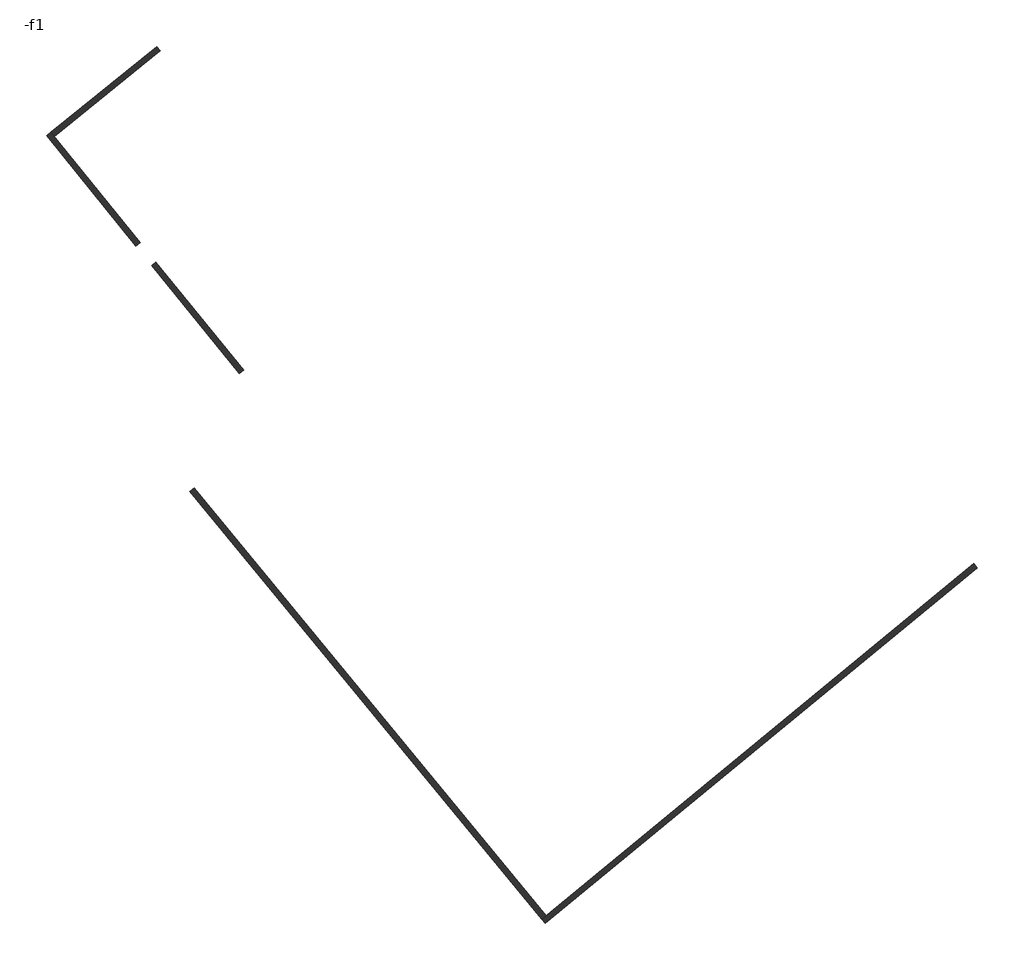
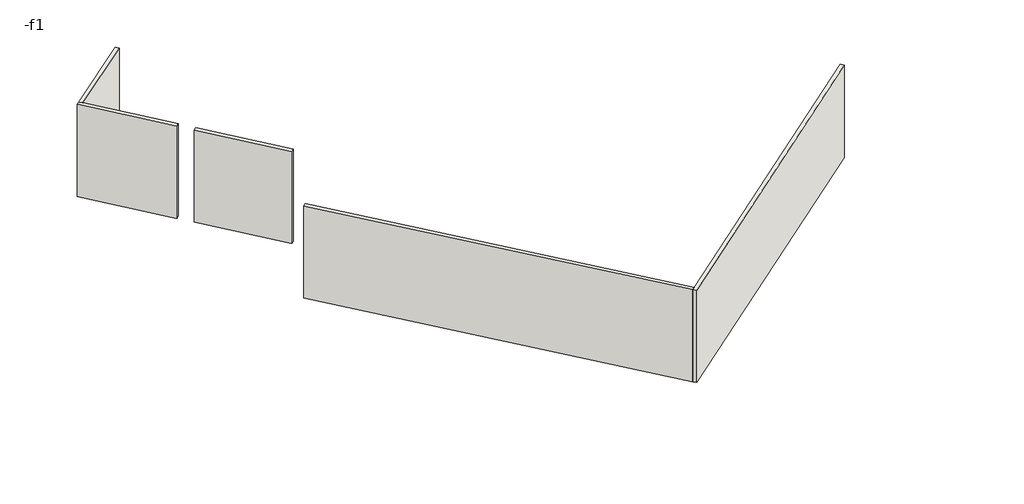
# One storey: 5 walls.
"""IFC4 building model written with IfcOpenShell, lengths in millimetres."""

from ifc_helpers import new_model, si_unit, frame, origin, place, context, project, spatial, polyline, outline, extrude, faceted_brep, element, save

model = new_model("IFC4")

# Units and contexts
model_context = context("Model", 3, world=origin())
ifc_project = project(units=[si_unit("LENGTHUNIT", "METRE", prefix="MILLI")], contexts=[model_context])

# Site, building, storey
site = spatial("IfcSite", under=ifc_project)
building = spatial("IfcBuilding", under=site)
storey = spatial("IfcBuildingStorey", under=building, Name="-f1", Elevation=-2300.0)

# Walls
placement = place(None, origin())
element("IfcWall", 1, ObjectType="aa-素混凝土-灰色 - 200mm", at=placement, inside=storey, context=model_context, shape_type="Brep", body=[
    faceted_brep([(-28826.4009096, -26995.4587154, -2300.0), (-13306.0693643, -14223.2502641, -2300.0), (-13306.0693643, -14223.2502641, 3100.0), (-28826.4009096, -26995.4587154, 3100.0), (-28953.4875609, -26841.0275558, -2300.0), (-28953.4875609, -26841.0275558, 3100.0), (-28799.0564012, -26713.9409045, 3100.0), (-13433.1560156, -14068.8191045, 3100.0), (-13433.1560156, -14068.8191045, -2300.0), (-28799.0564012, -26713.9409045, -2300.0)], [[[0, 1, 2, 3]], [[4, 5, 6, 7, 8, 9]], [[1, 0, 4, 9, 8]], [[2, 1, 8, 7]], [[3, 2, 7, 6, 5]], [[0, 3, 5, 4]]]),
])
element("IfcWall", 2, ObjectType="aa-素混凝土-灰色 - 200mm", at=placement, inside=storey, context=model_context, shape_type="SweptSolid", body=[
    extrude(outline(polyline([(-28953.4875609, -26841.0275558), (-41598.6093609, -11475.1271701), (-41444.1782013, -11348.0405189), (-28799.0564012, -26713.9409045), (-28953.4875609, -26841.0275558)])), frame((0.0, 0.0, -2300.0), z_axis=(0.0, 0.0, 1.0), x_axis=(1.0, 0.0, 0.0)), (0.0, 0.0, 1.0), 5400.0),
])
element("IfcWall", 3, ObjectType="aa-素混凝土-灰色 - 200mm", at=placement, inside=storey, context=model_context, shape_type="SweptSolid", body=[
    extrude(outline(polyline([(-39822.6602834, -7240.2562802), (-42969.2622386, -3354.5264729), (-42813.8330463, -3228.6623947), (-39667.2310911, -7114.392202), (-39822.6602834, -7240.2562802)])), frame((0.0, 0.0, -2300.0), z_axis=(0.0, 0.0, 1.0), x_axis=(1.0, 0.0, 0.0)), (0.0, 0.0, 1.0), 5400.0),
])
element("IfcWall", 4, ObjectType="aa-素混凝土-灰色 - 200mm", at=placement, inside=storey, context=model_context, shape_type="Brep", body=[
    faceted_brep([(-46745.1845849, 1308.3492958, -2300.0), (-43535.6505905, -2655.0951076, -2300.0), (-43535.6505905, -2655.0951076, 3100.0), (-46745.1845849, 1308.3492958, 3100.0), (-46589.7553926, 1434.2133741, -2300.0), (-46589.7553926, 1434.2133741, 3100.0), (-46463.8913144, 1278.7841818, 3100.0), (-43380.2213983, -2529.2310294, 3100.0), (-43380.2213983, -2529.2310294, -2300.0), (-46463.8913144, 1278.7841818, -2300.0)], [[[0, 1, 2, 3]], [[4, 5, 6, 7, 8, 9]], [[1, 0, 4, 9, 8]], [[2, 1, 8, 7]], [[3, 2, 7, 6, 5]], [[0, 3, 5, 4]]]),
])
element("IfcWall", 5, ObjectType="aa-素混凝土-灰色 - 200mm", at=placement, inside=storey, context=model_context, shape_type="SweptSolid", body=[
    extrude(outline(polyline([(-46589.7553926, 1434.2133741), (-42781.7401815, 4517.8832902), (-42655.8761033, 4362.4540979), (-46463.8913144, 1278.7841818), (-46589.7553926, 1434.2133741)])), frame((0.0, 0.0, -2300.0), z_axis=(0.0, 0.0, 1.0), x_axis=(1.0, 0.0, 0.0)), (0.0, 0.0, 1.0), 5400.0),
])

save(model, "model.ifc")

# Revit data of these elements
# Project information
#   项目发布日期 = "出图日期"
#   项目状态 = "项目状态"
#   客户姓名 = "所有者"
#   项目地址 = "请在此处输入地址"
#   项目名称 = "项目名称"
#   项目编号 = "项目编号"
# Type "aa-素混凝土-灰色 - 200mm"
#   Width = 200 mm
#   Layers, outside or top first: 200 mm "aa-素混凝土-灰色" (function 1)
# Elements 1, 2, 3, 4, 5 (IfcWall, "aa-素混凝土-灰色 - 200mm")
#   Top Offset = 0 mm
#   Base Offset = 0 mm
#   wall height = 5400 mm
#   Phase Created = 新构造
#   Base Constraint = -f1
#   Top Constraint = f1
#   Materials on its faces: "aa-素混凝土-灰色"
# Materials
#   "aa-素混凝土-灰色": class "混凝土", colour RGB 192 192 192, transparency 0
